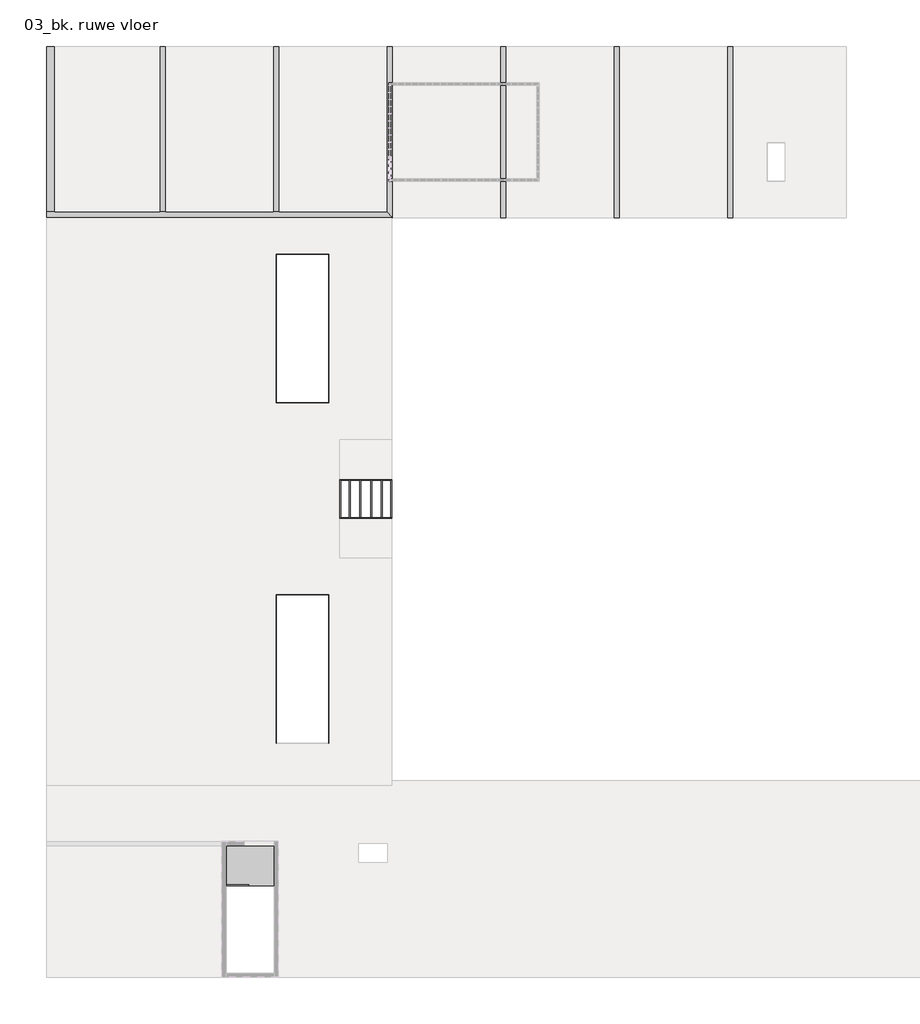
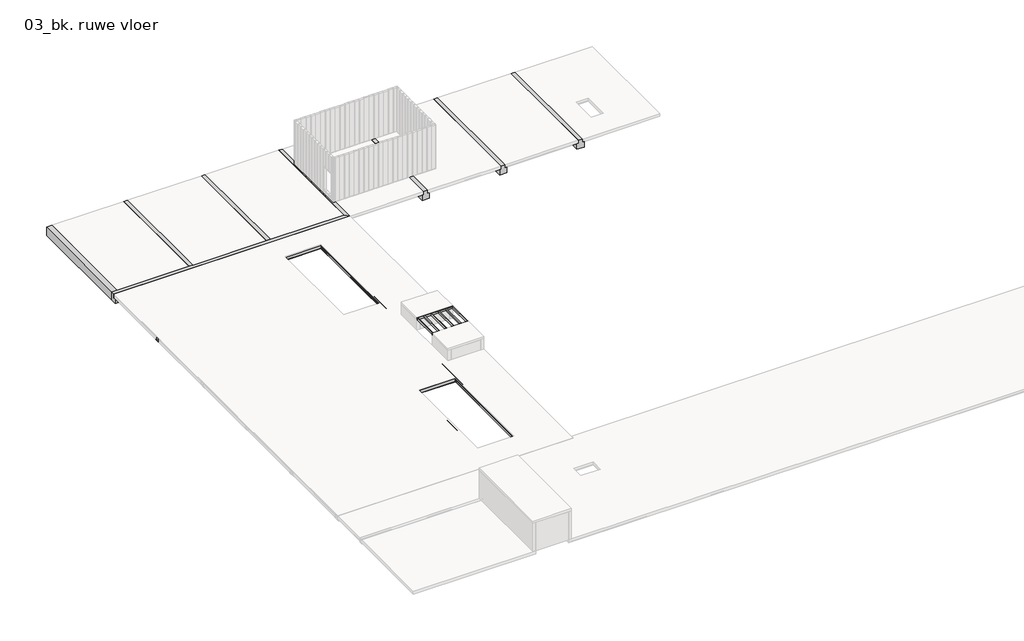
# One storey, part 9 of 9: 26 beams, 1 stair.
# Revit data of these elements (continued)
# Element 20 (IfcBeam, "NLRS_28_SF_LIB_stalen ligger HEB-AV-CWV-MMBS-SRP_gen_rsf : stalen ligger_gen__HEB 260") (continued)
#   LoadBearing = yes
#   Phase Created = NLRS_nieuw
#   Materials on its faces: "NLRS_h2_staal_gen_rsf"
# Element 21 (IfcBeam, "NLRS_28_SF_LIB_stalen ligger HEB-AV-CWV-MMBS-SRP_gen_rsf : stalen ligger_gen__HEB 260")
#   IfcGUID = "13lTCcCQ95UOWcvnmPh7D_"
#   Comments = ""
#   NLRS_C_lengte = 12637.5 mm
#   IsExternal = yes
#   LoadBearing = yes
#   Phase Created = NLRS_nieuw
#   Materials on its faces: "NLRS_h2_staal_gen_rsf"
# Element 22 (IfcBeam, "NLRS_28_SF_LIB_stalen ligger HEB-AV-CWV-MMBS-SRP_gen_rsf : stalen ligger_gen__HEB 260")
#   IfcGUID = "13lTCcCQ95UOWcvnmPh7Du"
#   Comments = ""
#   NLRS_C_lengte = 12637.5 mm
#   IsExternal = yes
#   LoadBearing = yes
#   Phase Created = NLRS_nieuw
#   Materials on its faces: "NLRS_h2_staal_gen_rsf"
# Element 23 (IfcBeam, "NLRS_28_SF_LIB_houten balk-MMBW-SRP_gen_rsf : houten balk_gen__bxh 58x156")
#   IfcGUID = "3PFmhy1jzBXho9jMrHR5Eo"
#   NLRS_C_lengte = 2250 mm
#   IsExternal = yes
#   LoadBearing = yes
#   Phase Created = NLRS_nieuw
#   Materials on its faces: "NLRS_i2_hout naaldhout vuren_gen_rsf"
# Element 24 (IfcBeam, "NLRS_28_SF_LIB_houten balk-MMBW-SRP_gen_rsf : houten balk_gen__bxh 58x156")
#   IfcGUID = "3PFmhy1jzBXho9jMrHR5Em"
#   NLRS_C_lengte = 2250 mm
#   IsExternal = yes
#   LoadBearing = yes
#   Phase Created = NLRS_nieuw
#   Materials on its faces: "NLRS_i2_hout naaldhout vuren_gen_rsf"
# Element 25 (IfcBeam, "NLRS_28_SF_LIB_houten balk-MMBW-SRP_gen_rsf : houten balk_gen__bxh 58x156")
#   IfcGUID = "3PFmhy1jzBXho9jMrHR5E_"
#   NLRS_C_lengte = 2250 mm
#   IsExternal = yes
#   LoadBearing = yes
#   Phase Created = NLRS_nieuw
#   Materials on its faces: "NLRS_i2_hout naaldhout vuren_gen_rsf"
# Element 26 (IfcBeam, "NLRS_28_SF_LIB_houten balk-MMBW-SRP_gen_rsf : houten balk_gen__bxh 58x156")
#   IfcGUID = "3PFmhy1jzBXho9jMrHR5Ey"
#   NLRS_C_lengte = 2250 mm
#   IsExternal = yes
#   LoadBearing = yes
#   Phase Created = NLRS_nieuw
#   Materials on its faces: "NLRS_i2_hout naaldhout vuren_gen_rsf"
# Element 27 (IfcStair, "NLRS_24_GM_UN_rechthoekig bordes prefab zonder oplegnok-AV_gen_rsf : prefab bordes_gen__2300x2730")
#   IfcGUID = "2CEqVLPNH8KRN7ghwV3apU"
#   IsExternal = no
#   LoadBearing = yes
#   Phase Created = NLRS_nieuw
#   Materials on its faces: "NLRS_f2_beton prefab_gen_rsf"
# Materials
#   "NLRS_f2_beton prefab_gen_rsf": class "F - Niet gebakken kunststeen", colour RGB 129 133 118, transparency 0, Keynote = "f2", Manufacturer = "Revit Standards Foundation", URL = "www.revitstandards.org", Description = "beton prefab", Cost = 0
#   "NLRS_i2_hout naaldhout vuren_gen_rsf": class "I - Hout", colour RGB 234 199 147, transparency 0, Keynote = "i2", Manufacturer = "Revit Standards Foundation", URL = "www.revitstandards.org", Description = "hout vuren", Cost = 0
#   "NLRS_h2_staal_gen_rsf": class "H - Metaal", colour RGB 189 187 185, transparency 0, Keynote = "h2", Manufacturer = "Revit Standards Foundation", URL = "www.revitstandards.org", Description = "staal", Cost = 0
